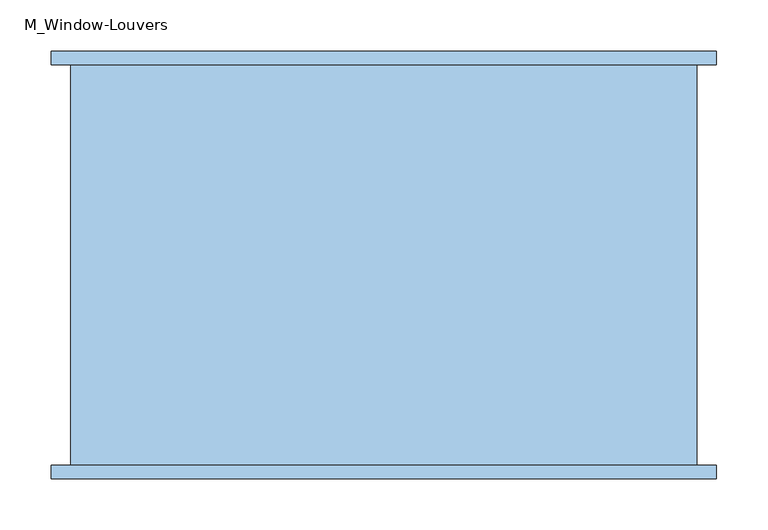
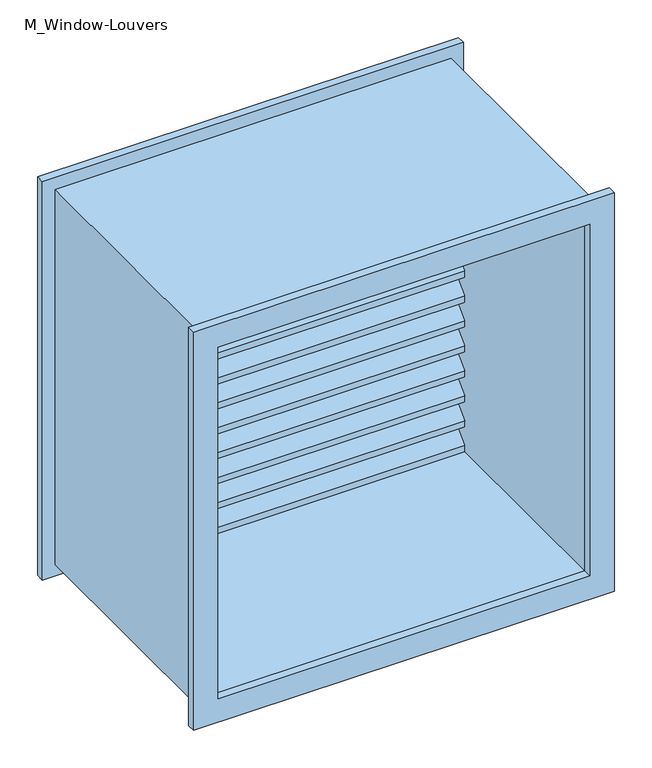
"""IFC4 building model written with IfcOpenShell, lengths in millimetres: window geometry, M_Window-Louvers : H_WD_AMW_AL Louver_W610xH610."""

from ifc_helpers import new_model, si_unit, frame, origin, place, context, project, spatial, polyline, outline, extrude, source, transform, mapped, element, save


def m_window_louvers_33c5b602(model_context):
    return source(origin(), model_context, "Body", "SweptSolid", [
        extrude(outline(polyline([(188.65, 1430.5146859), (188.65, 1420.4737696), (153.725, 1455.3987696), (118.8, 1420.4737696), (118.8, 1430.5146859), (153.725, 1465.4396859), (188.65, 1430.5146859)])), frame((-286.0, 0.0, 0.0), z_axis=(1.0, 0.0, 0.0), x_axis=(0.0, 1.0, 0.0)), (0.0, 0.0, 1.0), 572.0),
        extrude(outline(polyline([(188.65, 1389.9793717), (188.65, 1379.9384554), (153.725, 1414.8634554), (118.8, 1379.9384554), (118.8, 1389.9793717), (153.725, 1424.9043717), (188.65, 1389.9793717)])), frame((-286.0, 0.0, 0.0), z_axis=(1.0, 0.0, 0.0), x_axis=(0.0, 1.0, 0.0)), (0.0, 0.0, 1.0), 572.0),
        extrude(outline(polyline([(188.65, 1349.4440576), (188.65, 1339.4031413), (153.725, 1374.3281413), (118.8, 1339.4031413), (118.8, 1349.4440576), (153.725, 1384.3690576), (188.65, 1349.4440576)])), frame((-286.0, 0.0, 0.0), z_axis=(1.0, 0.0, 0.0), x_axis=(0.0, 1.0, 0.0)), (0.0, 0.0, 1.0), 572.0),
        extrude(outline(polyline([(188.65, 1308.9087435), (188.65, 1298.8678272), (153.725, 1333.7928272), (118.8, 1298.8678272), (118.8, 1308.9087435), (153.725, 1343.8337435), (188.65, 1308.9087435)])), frame((-286.0, 0.0, 0.0), z_axis=(1.0, 0.0, 0.0), x_axis=(0.0, 1.0, 0.0)), (0.0, 0.0, 1.0), 572.0),
        extrude(outline(polyline([(188.65, 1268.3734293), (188.65, 1258.3325131), (153.725, 1293.2575131), (118.8, 1258.3325131), (118.8, 1268.3734293), (153.725, 1303.2984293), (188.65, 1268.3734293)])), frame((-286.0, 0.0, 0.0), z_axis=(1.0, 0.0, 0.0), x_axis=(0.0, 1.0, 0.0)), (0.0, 0.0, 1.0), 572.0),
        extrude(outline(polyline([(188.65, 1227.8381152), (188.65, 1217.7971989), (153.725, 1252.7221989), (118.8, 1217.7971989), (118.8, 1227.8381152), (153.725, 1262.7631152), (188.65, 1227.8381152)])), frame((-286.0, 0.0, 0.0), z_axis=(1.0, 0.0, 0.0), x_axis=(0.0, 1.0, 0.0)), (0.0, 0.0, 1.0), 572.0),
        extrude(outline(polyline([(188.65, 1187.3028011), (188.65, 1177.2618848), (153.725, 1212.1868848), (118.8, 1177.2618848), (118.8, 1187.3028011), (153.725, 1222.2278011), (188.65, 1187.3028011)])), frame((-286.0, 0.0, 0.0), z_axis=(1.0, 0.0, 0.0), x_axis=(0.0, 1.0, 0.0)), (0.0, 0.0, 1.0), 572.0),
        extrude(outline(polyline([(188.65, 1146.7674869), (188.65, 1136.7265707), (153.725, 1171.6515707), (118.8, 1136.7265707), (118.8, 1146.7674869), (153.725, 1181.6924869), (188.65, 1146.7674869)])), frame((-286.0, 0.0, 0.0), z_axis=(1.0, 0.0, 0.0), x_axis=(0.0, 1.0, 0.0)), (0.0, 0.0, 1.0), 572.0),
        extrude(outline(polyline([(188.65, 1106.2321728), (188.65, 1096.1912565), (153.725, 1131.1162565), (118.8, 1096.1912565), (118.8, 1106.2321728), (153.725, 1141.1571728), (188.65, 1106.2321728)])), frame((-286.0, 0.0, 0.0), z_axis=(1.0, 0.0, 0.0), x_axis=(0.0, 1.0, 0.0)), (0.0, 0.0, 1.0), 572.0),
        extrude(outline(polyline([(188.65, 1065.6968587), (188.65, 1055.6559424), (153.725, 1090.5809424), (118.8, 1055.6559424), (118.8, 1065.6968587), (153.725, 1100.6218587), (188.65, 1065.6968587)])), frame((-286.0, 0.0, 0.0), z_axis=(1.0, 0.0, 0.0), x_axis=(0.0, 1.0, 0.0)), (0.0, 0.0, 1.0), 572.0),
        extrude(outline(polyline([(188.65, 1025.1615446), (188.65, 1015.1206283), (153.725, 1050.0456283), (118.8, 1015.1206283), (118.8, 1025.1615446), (153.725, 1060.0865446), (188.65, 1025.1615446)])), frame((-286.0, 0.0, 0.0), z_axis=(1.0, 0.0, 0.0), x_axis=(0.0, 1.0, 0.0)), (0.0, 0.0, 1.0), 572.0),
        extrude(outline(polyline([(188.65, 984.6262304), (188.65, 974.5853141), (153.725, 1009.5103141), (118.8, 974.5853141), (118.8, 984.6262304), (153.725, 1019.5512304), (188.65, 984.6262304)])), frame((-286.0, 0.0, 0.0), z_axis=(1.0, 0.0, 0.0), x_axis=(0.0, 1.0, 0.0)), (0.0, 0.0, 1.0), 572.0),
        extrude(outline(polyline([(188.65, 1471.05), (188.65, 1461.0090837), (153.725, 1495.9340837), (118.8, 1461.0090837), (118.8, 1471.05), (153.725, 1505.975), (188.65, 1471.05)])), frame((-286.0, 0.0, 0.0), z_axis=(1.0, 0.0, 0.0), x_axis=(0.0, 1.0, 0.0)), (0.0, 0.0, 1.0), 572.0),
        extrude(outline(polyline([(188.65, 944.0909163), (188.65, 934.05), (153.725, 968.975), (118.8, 934.05), (118.8, 944.0909163), (153.725, 979.0159163), (188.65, 944.0909163)])), frame((-286.0, 0.0, 0.0), z_axis=(1.0, 0.0, 0.0), x_axis=(0.0, 1.0, 0.0)), (0.0, 0.0, 1.0), 572.0),
        extrude(outline(polyline([(1543.975, -323.95), (896.05, -323.95), (896.05, 323.95), (1543.975, 323.95), (1543.975, -323.95)]), holes=[polyline([(1505.95, -285.95), (1505.95, 285.95), (934.05, 285.95), (934.05, -285.95), (1505.95, -285.95)])]), frame((0.0, 188.65, 0.0), z_axis=(0.0, 1.0, 0.0), x_axis=(0.0, 0.0, 1.0)), (0.0, 0.0, 1.0), 13.0),
        extrude(outline(polyline([(1543.975, 323.95), (1543.975, -323.95), (896.05, -323.95), (896.05, 323.95), (1543.975, 323.95)]), holes=[polyline([(1505.975, 285.95), (934.05, 285.95), (934.05, -285.95), (1505.975, -285.95), (1505.975, 285.95)])]), frame((0.0, -214.35, 0.0), z_axis=(0.0, 1.0, 0.0), x_axis=(0.0, 0.0, 1.0)), (0.0, 0.0, 1.0), 13.0),
        extrude(outline(polyline([(1525.0, 305.0), (1525.0, -305.0), (915.0, -305.0), (915.0, 305.0), (1525.0, 305.0)]), holes=[polyline([(1505.95, 285.95), (934.05, 285.95), (934.05, -285.95), (1505.95, -285.95), (1505.95, 285.95)])]), frame((0.0, -201.35, 0.0), z_axis=(0.0, 1.0, 0.0), x_axis=(0.0, 0.0, 1.0)), (0.0, 0.0, 1.0), 390.0),
    ])


if __name__ == "__main__":
    model = new_model("IFC4")
    model_context = context("Model", 3, world=origin())
    ifc_project = project(units=[si_unit("LENGTHUNIT", "METRE", prefix="MILLI")], contexts=[model_context])
    site = spatial("IfcSite", under=ifc_project)
    building = spatial("IfcBuilding", under=site)
    placement = place(None, origin())
    m_window_louvers_shape = m_window_louvers_33c5b602(model_context)
    element("IfcWindow", 1, ObjectType="M_Window-Louvers : H_WD_AMW_AL Louver_W610xH610", at=placement, inside=building, context=model_context, shape_type="MappedRepresentation", body=[
        mapped(m_window_louvers_shape, transform((0.0, 0.0, 0.0), x_axis=(1.0, 0.0, 0.0), y_axis=(0.0, 1.0, 0.0), z_axis=(0.0, 0.0, 1.0))),
    ])
    save(model, "model.ifc")

# Revit data of these elements
# Type "M_Window-Louvers : H_WD_AMW_AL Louver_W610xH610"
#   Type Mark = "AL"
#   Construction Type Id = "GSP4R"
#   Analytic Construction = "1/8 in Pilkington single glazing"
#   Visual Light Transmittance = 0.9
#   Thermal Resistance (R) = 0.271106 (m²·K)/W
#   Solar Heat Gain Coefficient = 0.78
#   Max Height = 0.603598 m
#   Height = 0.6100 m
#   Heat Transfer Coefficient (U) = 3.6886 W/(m²·K)
#   Default Sill Height = 0.9150 m
#   Trim Projection_Exterior = 0.0130 m
#   Trim Projection_Interior = 0.0130 m
#   Trim Width_Exterior = 0.0380 m
#   Trim Width_Interior = 0.0380 m
#   Width = 0.6100 m
#   Blade Width = 0.5720 m
#   Blade Vertical Thickness = 0.010041 m
#   Blade Thickness = 0.0071 m
#   Blade Spacing = 0.0300 m
#   Blade Height = 0.044966 m
#   Blade Depth = 0.06985 m
#   Blade Angle = 45.00°
#   Max Blade Count = 14
#   Define Thermal Properties by = 1
#   Blade Count = 14
#   Frame Material = Birch
#   Louvers Material = Birch
#   Trim Exterior Material = Birch
#   Trim Interior Material = Birch
#   Wall Closure = (empty or 0)
# Element 1 (IfcWindow, "M_Window-Louvers : H_WD_AMW_AL Louver_W610xH610")
#   Materials on its faces: "Birch"
# Materials
#   "Birch": class "Wood", colour RGB 224 178 126, transparency 0, Description = "Betula Alleghaniensis", Cost = 0
